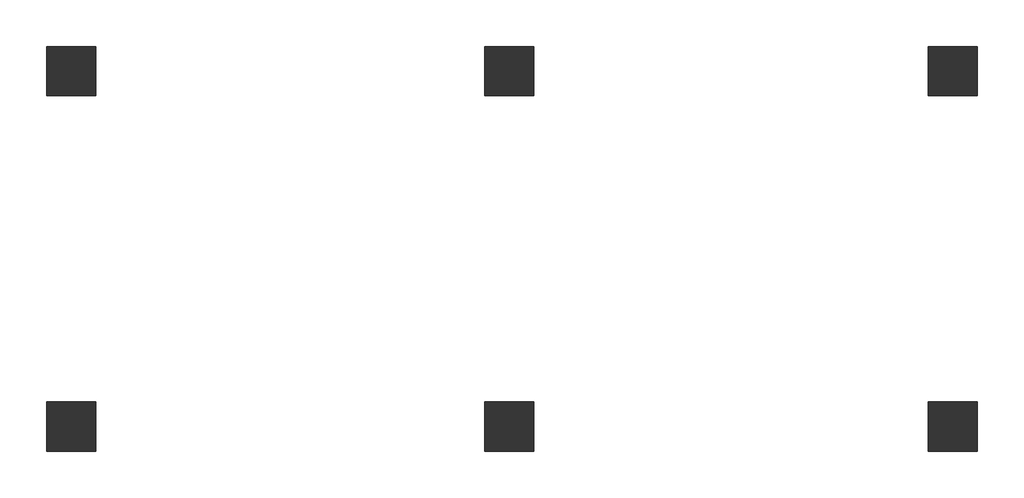
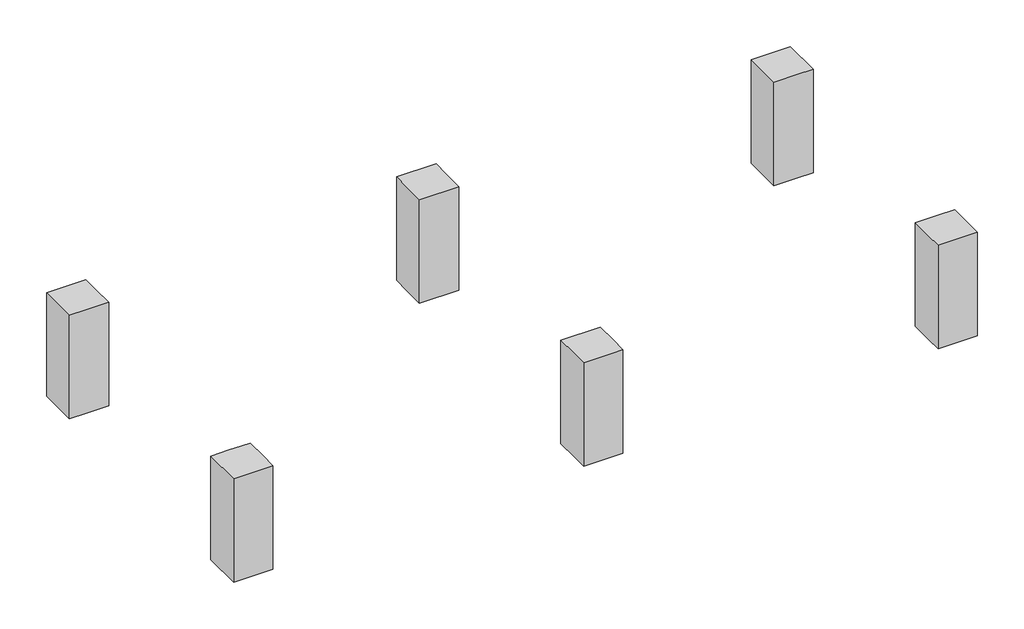
# One storey: 6 columns.
"""IFC4 building model written with IfcOpenShell, lengths in millimetres."""

from ifc_helpers import new_model, si_unit, origin, place, context, project, spatial, faceted_brep, element, save

model = new_model("IFC4")

# Units and contexts
model_context = context("Model", 3, world=origin())
ifc_project = project(units=[si_unit("LENGTHUNIT", "METRE", prefix="MILLI")], contexts=[model_context])

# Site, building, storey
site = spatial("IfcSite", under=ifc_project)
building = spatial("IfcBuilding", under=site)
storey = spatial("IfcBuildingStorey", under=building, Name="T.O.C", Elevation=-1900.0279945)

# Columns
placement = place(None, origin())
element("IfcColumn", 1, ObjectType="RC_Pedestal : H_SC_ACC_PED_W900xL900", at=placement, inside=storey, context=model_context, shape_type="Brep", body=[
    faceted_brep([(10680.0, 34449.5208589, -1900.0279945), (10680.0, 34059.5208589, -1900.0279945), (10680.0, 33549.5208589, -1900.0279945), (10170.0, 33549.5208589, -1900.0279945), (9780.0, 33549.5208589, -1900.0279945), (9780.0, 34449.5208589, -1900.0279945), (10680.0, 34449.5208589, 599.9720055), (10680.0, 34059.5208589, 599.9720055), (10680.0, 33549.5208589, 599.9720055), (10170.0, 33549.5208589, 599.9720055), (9780.0, 33549.5208589, 599.9720055), (9780.0, 34449.5208589, 599.9720055)], [[[0, 1, 2, 3, 4, 5]], [[6, 7, 8, 2, 1, 0]], [[8, 9, 10, 4, 3, 2]], [[10, 11, 5, 4]], [[11, 6, 0, 5]], [[6, 11, 10, 9, 8, 7]]]),
])
element("IfcColumn", 2, ObjectType="RC_Pedestal : H_SC_ACC_PED_W900xL900", at=placement, inside=storey, context=model_context, shape_type="Brep", body=[
    faceted_brep([(10680.0, 27949.5208589, -1900.0279945), (10680.0, 27439.5208589, -1900.0279945), (10680.0, 27049.5208589, -1900.0279945), (9780.0, 27049.5208589, -1900.0279945), (9780.0, 27949.5208589, -1900.0279945), (10170.0, 27949.5208589, -1900.0279945), (10680.0, 27949.5208589, 599.9720055), (10680.0, 27439.5208589, 599.9720055), (10680.0, 27049.5208589, 599.9720055), (9780.0, 27049.5208589, 599.9720055), (9780.0, 27949.5208589, 599.9720055), (10170.0, 27949.5208589, 599.9720055)], [[[0, 1, 2, 3, 4, 5]], [[6, 7, 8, 2, 1, 0]], [[8, 9, 3, 2]], [[9, 10, 4, 3]], [[10, 11, 6, 0, 5, 4]], [[6, 11, 10, 9, 8, 7]]]),
])
element("IfcColumn", 3, ObjectType="RC_Pedestal : H_SC_ACC_PED_W900xL900", at=placement, inside=storey, context=model_context, shape_type="Brep", body=[
    faceted_brep([(26780.0, 34449.5208589, -1900.0279945), (26780.0, 33549.5208589, -1900.0279945), (26390.0, 33549.5208589, -1900.0279945), (25880.0, 33549.5208589, -1900.0279945), (25880.0, 34059.5208589, -1900.0279945), (25880.0, 34449.5208589, -1900.0279945), (26780.0, 34449.5208589, 599.9720055), (26780.0, 33549.5208589, 599.9720055), (26390.0, 33549.5208589, 599.9720055), (25880.0, 33549.5208589, 599.9720055), (25880.0, 34059.5208589, 599.9720055), (25880.0, 34449.5208589, 599.9720055)], [[[0, 1, 2, 3, 4, 5]], [[6, 7, 1, 0]], [[7, 8, 9, 3, 2, 1]], [[9, 10, 11, 5, 4, 3]], [[11, 6, 0, 5]], [[6, 11, 10, 9, 8, 7]]]),
])
element("IfcColumn", 4, ObjectType="RC_Pedestal : H_SC_ACC_PED_W900xL900", at=placement, inside=storey, context=model_context, shape_type="Brep", body=[
    faceted_brep([(26780.0, 27949.5208589, -1900.0279945), (26780.0, 27049.5208589, -1900.0279945), (25880.0, 27049.5208589, -1900.0279945), (25880.0, 27439.5208589, -1900.0279945), (25880.0, 27949.5208589, -1900.0279945), (26390.0, 27949.5208589, -1900.0279945), (26780.0, 27949.5208589, 599.9720055), (26780.0, 27049.5208589, 599.9720055), (25880.0, 27049.5208589, 599.9720055), (25880.0, 27439.5208589, 599.9720055), (25880.0, 27949.5208589, 599.9720055), (26390.0, 27949.5208589, 599.9720055)], [[[0, 1, 2, 3, 4, 5]], [[6, 7, 1, 0]], [[7, 8, 2, 1]], [[8, 9, 10, 4, 3, 2]], [[10, 11, 6, 0, 5, 4]], [[6, 11, 10, 9, 8, 7]]]),
])
element("IfcColumn", 5, ObjectType="RC_Pedestal : H_SC_ACC_PED_W900xL900", at=placement, inside=storey, context=model_context, shape_type="Brep", body=[
    faceted_brep([(18680.0, 34449.5208589, -1900.0279945), (18680.0, 34059.5208589, -1900.0279945), (18680.0, 33549.5208589, -1900.0279945), (17780.0, 33549.5208589, -1900.0279945), (17780.0, 34059.5208589, -1900.0279945), (17780.0, 34449.5208589, -1900.0279945), (18680.0, 34449.5208589, 599.9720055), (18680.0, 34059.5208589, 599.9720055), (18680.0, 33549.5208589, 599.9720055), (17780.0, 33549.5208589, 599.9720055), (17780.0, 34059.5208589, 599.9720055), (17780.0, 34449.5208589, 599.9720055)], [[[0, 1, 2, 3, 4, 5]], [[6, 7, 8, 2, 1, 0]], [[8, 9, 3, 2]], [[9, 10, 11, 5, 4, 3]], [[11, 6, 0, 5]], [[6, 11, 10, 9, 8, 7]]]),
])
element("IfcColumn", 6, ObjectType="RC_Pedestal : H_SC_ACC_PED_W900xL900", at=placement, inside=storey, context=model_context, shape_type="Brep", body=[
    faceted_brep([(18680.0, 27949.5208589, -1900.0279945), (18680.0, 27439.5208589, -1900.0279945), (18680.0, 27049.5208589, -1900.0279945), (17780.0, 27049.5208589, -1900.0279945), (17780.0, 27439.5208589, -1900.0279945), (17780.0, 27949.5208589, -1900.0279945), (18680.0, 27949.5208589, 599.9720055), (18680.0, 27439.5208589, 599.9720055), (18680.0, 27049.5208589, 599.9720055), (17780.0, 27049.5208589, 599.9720055), (17780.0, 27439.5208589, 599.9720055), (17780.0, 27949.5208589, 599.9720055)], [[[0, 1, 2, 3, 4, 5]], [[6, 7, 8, 2, 1, 0]], [[8, 9, 3, 2]], [[9, 10, 11, 5, 4, 3]], [[11, 6, 0, 5]], [[6, 11, 10, 9, 8, 7]]]),
])

save(model, "model.ifc")

# Revit data of these elements
# Type "RC_Pedestal : H_SC_ACC_PED_W900xL900"
#   H_WM Code_1 = "A03AD032-00012 | Concrete Work | Substructure Work | Structural Concrete | Cement Type-5 | 20MPa < F'c (Cylinder Strength) ≤ 25MPa"
#   H_WM Code_2 = "A03AD037-00002 | Concrete Work | Substructure Work | Rebar Work | Deformed Bar (Non-Coat.) | 400MPa<Fy≤470MPa"
#   H_WM Code_3 = "A03AD035-00001 | Concrete Work | Substructure Work | Form Work (3 times in use) | Flat Form | Dressed Lumber, Plywood or Steel Form(Wood Planks are not Allowed) incl. Chamfer"
#   H_WM Code_4 = "A03AH056-00001 | Concrete Work | Concrete Protective Coating (U/G) | Bitumen/Bituminous/Asphalt Coating"
#   H_Q'ty Cal Type Tag = "SC-Q1"
#   Description = "AG RC 기둥"
#   Width = 0.9000 m
#   Length = 0.9000 m
#   hec_material3 [instance default] = none
#   hec_material2 [instance default] = A04AM078-00002_Int Wall Painting_Water Emulsion Paint
#   hec_material1 [instance default] = A03AD036-00001_Form Work (1 time in use)
#   Structural Material [instance default] = A03AD032-00007_Structural Concrete_25MPa-30MPa
# Elements 1, 2, 3, 4, 5, 6 (IfcColumn, "RC_Pedestal : H_SC_ACC_PED_W900xL900")
#   Mark = "C1"
#   hec_material3 = none
#   hec_material2 = none
#   hec_material1 = none
#   Structural Material = A03AG034-00004_Mass Concrete_Structural Concrete_Type-1_30MPa-35Mpa
#   Phase Created = New Construction
#   Materials on its faces: "A03AG034-00004_Mass Concrete_Structural Concrete_Type-1_30MPa-35Mpa"
# Materials
#   "A04AM078-00002_Int Wall Painting_Water Emulsion Paint": class "Paint", colour RGB 128 128 64, transparency 0, Description = "Finishing Work / Painting Work / Internal Wall Painting / Water Emulsion Paint", Cost = 0
#   "A03AD036-00001_Form Work (1 time in use)": class "Wood", colour RGB 149 120 74, transparency 0, Description = "Plywood", Cost = 0
#   "A03AD032-00007_Structural Concrete_25MPa-30MPa": class "Concrete", colour RGB 176 176 176, transparency 0, Keynote = "09910.A1", Description = "LATEX PAINT ON F.F CONC.", Cost = 0
#   "A03AG034-00004_Mass Concrete_Structural Concrete_Type-1_30MPa-35Mpa": class "Concrete", colour RGB 176 176 176, transparency 0, Keynote = "09910.A1", Description = "Reinf. Conc.", Cost = 0
